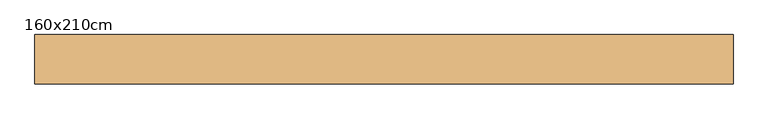
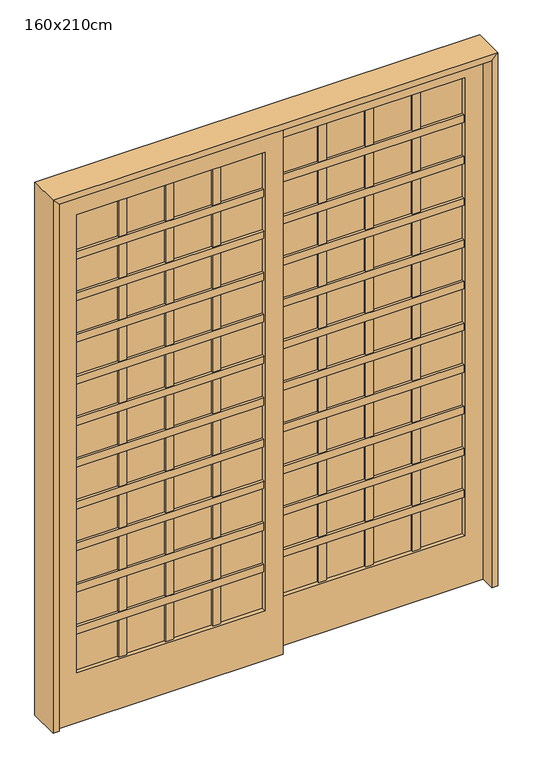
"""IFC4 building model written with IfcOpenShell, lengths in millimetres: door geometry, Porta de Correr Metálica Quadriculada : 160x210cm."""

from ifc_helpers import new_model, si_unit, frame, origin, place, context, project, spatial, polyline, outline, extrude, faceted_brep, source, transform, mapped, element, save


def door_160x210cm_3b8a9287(model_context):
    return source(origin(), model_context, "Body", "SolidModel", [
        extrude(outline(polyline([(-199.5, -52.1), (-199.5, -67.1101935), (-229.5, -67.1101935), (-229.5, -52.1), (-199.5, -52.1)])), frame((0.0, 0.0, 253.0), z_axis=(0.0, 0.0, 1.0), x_axis=(1.0, 0.0, 0.0)), (0.0, 0.0, 1.0), 1850.0),
        extrude(outline(polyline([(-379.0, -52.1), (-379.0, -67.1101935), (-409.0, -67.1101935), (-409.0, -52.1), (-379.0, -52.1)])), frame((0.0, 0.0, 253.0), z_axis=(0.0, 0.0, 1.0), x_axis=(1.0, 0.0, 0.0)), (0.0, 0.0, 1.0), 1850.0),
        extrude(outline(polyline([(-558.5, -52.1), (-558.5, -67.1101935), (-588.5, -67.1101935), (-588.5, -52.1), (-558.5, -52.1)])), frame((0.0, 0.0, 253.0), z_axis=(0.0, 0.0, 1.0), x_axis=(1.0, 0.0, 0.0)), (0.0, 0.0, 1.0), 1850.0),
        extrude(outline(polyline([(-35.0, -49.1), (-35.0, -70.1), (-753.0, -70.1), (-753.0, -49.1), (-35.0, -49.1)])), frame((0.0, 0.0, 1415.2727273), z_axis=(0.0, 0.0, 1.0), x_axis=(1.0, 0.0, 0.0)), (0.0, 0.0, 1.0), 30.0),
        extrude(outline(polyline([(-35.0, -49.1), (-35.0, -70.1), (-753.0, -70.1), (-753.0, -49.1), (-35.0, -49.1)])), frame((0.0, 0.0, 1247.0909091), z_axis=(0.0, 0.0, 1.0), x_axis=(1.0, 0.0, 0.0)), (0.0, 0.0, 1.0), 30.0),
        extrude(outline(polyline([(-35.0, -49.1), (-35.0, -70.1), (-753.0, -70.1), (-753.0, -49.1), (-35.0, -49.1)])), frame((0.0, 0.0, 1078.9090909), z_axis=(0.0, 0.0, 1.0), x_axis=(1.0, 0.0, 0.0)), (0.0, 0.0, 1.0), 30.0),
        extrude(outline(polyline([(-35.0, -49.1), (-35.0, -70.1), (-753.0, -70.1), (-753.0, -49.1), (-35.0, -49.1)])), frame((0.0, 0.0, 910.7272727), z_axis=(0.0, 0.0, 1.0), x_axis=(1.0, 0.0, 0.0)), (0.0, 0.0, 1.0), 30.0),
        extrude(outline(polyline([(-35.0, -49.1), (-35.0, -70.1), (-753.0, -70.1), (-753.0, -49.1), (-35.0, -49.1)])), frame((0.0, 0.0, 742.5454545), z_axis=(0.0, 0.0, 1.0), x_axis=(1.0, 0.0, 0.0)), (0.0, 0.0, 1.0), 30.0),
        extrude(outline(polyline([(-35.0, -49.1), (-35.0, -70.1), (-753.0, -70.1), (-753.0, -49.1), (-35.0, -49.1)])), frame((0.0, 0.0, 574.3636364), z_axis=(0.0, 0.0, 1.0), x_axis=(1.0, 0.0, 0.0)), (0.0, 0.0, 1.0), 30.0),
        extrude(outline(polyline([(-35.0, -49.1), (-35.0, -70.1), (-753.0, -70.1), (-753.0, -49.1), (-35.0, -49.1)])), frame((0.0, 0.0, 406.1818182), z_axis=(0.0, 0.0, 1.0), x_axis=(1.0, 0.0, 0.0)), (0.0, 0.0, 1.0), 30.0),
        extrude(outline(polyline([(-35.0, -49.1), (-35.0, -70.1), (-753.0, -70.1), (-753.0, -49.1), (-35.0, -49.1)])), frame((0.0, 0.0, 1919.8181818), z_axis=(0.0, 0.0, 1.0), x_axis=(1.0, 0.0, 0.0)), (0.0, 0.0, 1.0), 30.0),
        extrude(outline(polyline([(-35.0, -49.1), (-35.0, -70.1), (-753.0, -70.1), (-753.0, -49.1), (-35.0, -49.1)])), frame((0.0, 0.0, 1751.6363636), z_axis=(0.0, 0.0, 1.0), x_axis=(1.0, 0.0, 0.0)), (0.0, 0.0, 1.0), 30.0),
        extrude(outline(polyline([(-35.0, -49.1), (-35.0, -70.1), (-753.0, -70.1), (-753.0, -49.1), (-35.0, -49.1)])), frame((0.0, 0.0, 1583.4545455), z_axis=(0.0, 0.0, 1.0), x_axis=(1.0, 0.0, 0.0)), (0.0, 0.0, 1.0), 30.0),
        extrude(outline(polyline([(588.5, -10.1), (588.5, -25.1), (558.5, -25.1), (558.5, -10.1), (588.5, -10.1)])), frame((0.0, 0.0, 253.0), z_axis=(0.0, 0.0, 1.0), x_axis=(1.0, 0.0, 0.0)), (0.0, 0.0, 1.0), 1850.0),
        extrude(outline(polyline([(409.0, -10.1), (409.0, -25.1), (379.0, -25.1), (379.0, -10.1), (409.0, -10.1)])), frame((0.0, 0.0, 253.0), z_axis=(0.0, 0.0, 1.0), x_axis=(1.0, 0.0, 0.0)), (0.0, 0.0, 1.0), 1850.0),
        extrude(outline(polyline([(229.5, -10.1), (229.5, -25.1), (199.5, -25.1), (199.5, -10.1), (229.5, -10.1)])), frame((0.0, 0.0, 253.0), z_axis=(0.0, 0.0, 1.0), x_axis=(1.0, 0.0, 0.0)), (0.0, 0.0, 1.0), 1850.0),
        extrude(outline(polyline([(753.0, -7.1), (753.0, -28.1), (35.0, -28.1), (35.0, -7.1), (753.0, -7.1)])), frame((0.0, 0.0, 1415.2727273), z_axis=(0.0, 0.0, 1.0), x_axis=(1.0, 0.0, 0.0)), (0.0, 0.0, 1.0), 30.0),
        extrude(outline(polyline([(753.0, -7.1), (753.0, -28.1), (35.0, -28.1), (35.0, -7.1), (753.0, -7.1)])), frame((0.0, 0.0, 1247.0909091), z_axis=(0.0, 0.0, 1.0), x_axis=(1.0, 0.0, 0.0)), (0.0, 0.0, 1.0), 30.0),
        extrude(outline(polyline([(753.0, -7.1), (753.0, -28.1), (35.0, -28.1), (35.0, -7.1), (753.0, -7.1)])), frame((0.0, 0.0, 1078.9090909), z_axis=(0.0, 0.0, 1.0), x_axis=(1.0, 0.0, 0.0)), (0.0, 0.0, 1.0), 30.0),
        extrude(outline(polyline([(753.0, -7.1), (753.0, -28.1), (35.0, -28.1), (35.0, -7.1), (753.0, -7.1)])), frame((0.0, 0.0, 910.7272727), z_axis=(0.0, 0.0, 1.0), x_axis=(1.0, 0.0, 0.0)), (0.0, 0.0, 1.0), 30.0),
        extrude(outline(polyline([(753.0, -7.1), (753.0, -28.1), (35.0, -28.1), (35.0, -7.1), (753.0, -7.1)])), frame((0.0, 0.0, 742.5454545), z_axis=(0.0, 0.0, 1.0), x_axis=(1.0, 0.0, 0.0)), (0.0, 0.0, 1.0), 30.0),
        extrude(outline(polyline([(753.0, -7.1), (753.0, -28.1), (35.0, -28.1), (35.0, -7.1), (753.0, -7.1)])), frame((0.0, 0.0, 574.3636364), z_axis=(0.0, 0.0, 1.0), x_axis=(1.0, 0.0, 0.0)), (0.0, 0.0, 1.0), 30.0),
        extrude(outline(polyline([(753.0, -7.1), (753.0, -28.1), (35.0, -28.1), (35.0, -7.1), (753.0, -7.1)])), frame((0.0, 0.0, 406.1818182), z_axis=(0.0, 0.0, 1.0), x_axis=(1.0, 0.0, 0.0)), (0.0, 0.0, 1.0), 30.0),
        extrude(outline(polyline([(753.0, -7.1), (753.0, -28.1), (35.0, -28.1), (35.0, -7.1), (753.0, -7.1)])), frame((0.0, 0.0, 1919.8181818), z_axis=(0.0, 0.0, 1.0), x_axis=(1.0, 0.0, 0.0)), (0.0, 0.0, 1.0), 30.0),
        extrude(outline(polyline([(753.0, -7.1), (753.0, -28.1), (35.0, -28.1), (35.0, -7.1), (753.0, -7.1)])), frame((0.0, 0.0, 1751.6363636), z_axis=(0.0, 0.0, 1.0), x_axis=(1.0, 0.0, 0.0)), (0.0, 0.0, 1.0), 30.0),
        extrude(outline(polyline([(753.0, -7.1), (753.0, -28.1), (35.0, -28.1), (35.0, -7.1), (753.0, -7.1)])), frame((0.0, 0.0, 1583.4545455), z_axis=(0.0, 0.0, 1.0), x_axis=(1.0, 0.0, 0.0)), (0.0, 0.0, 1.0), 30.0),
        extrude(outline(polyline([(2173.0, -35.0), (53.0, -35.0), (53.0, 823.0), (2173.0, 823.0), (2173.0, -35.0)]), holes=[polyline([(2103.0, 35.0), (2103.0, 753.0), (253.0, 753.0), (253.0, 35.0), (2103.0, 35.0)])]), frame((0.0, -33.6, 0.0), z_axis=(0.0, 1.0, 0.0), x_axis=(0.0, 0.0, 1.0)), (0.0, 0.0, 1.0), 32.0),
        faceted_brep([(-826.0, -85.6, 50.0), (-850.0, -85.6, 50.0), (-850.0, 34.4, 50.0), (-826.0, 34.4, 50.0), (-826.0, 34.4, 2176.0), (-826.0, -85.6, 2176.0), (-850.0, 34.4, 2200.0), (-850.0, -85.6, 2200.0), (826.0, -85.6, 50.0), (826.0, 34.4, 50.0), (850.0, 34.4, 50.0), (850.0, -85.6, 50.0), (826.0, -85.6, 2176.0), (850.0, -85.6, 2200.0), (850.0, 34.4, 2200.0), (826.0, 34.4, 2176.0)], [[[0, 1, 2, 3]], [[3, 4, 5, 0]], [[2, 6, 4, 3]], [[1, 7, 6, 2]], [[0, 5, 7, 1]], [[8, 9, 10, 11]], [[12, 8, 11, 13]], [[13, 11, 10, 14]], [[14, 10, 9, 15]], [[15, 9, 8, 12]], [[4, 15, 12, 5]], [[6, 14, 15, 4]], [[7, 13, 14, 6]], [[5, 12, 13, 7]]]),
        extrude(outline(polyline([(2173.0, -823.0), (53.0, -823.0), (53.0, 35.0), (2173.0, 35.0), (2173.0, -823.0)]), holes=[polyline([(2103.0, -753.0), (2103.0, -35.0), (253.0, -35.0), (253.0, -753.0), (2103.0, -753.0)])]), frame((0.0, -75.6, 0.0), z_axis=(0.0, 1.0, 0.0), x_axis=(0.0, 0.0, 1.0)), (0.0, 0.0, 1.0), 32.0),
        extrude(outline(polyline([(-35.0, -54.1), (-35.0, -60.1), (-753.0, -60.1), (-753.0, -54.1), (-35.0, -54.1)])), frame((0.0, 0.0, 253.0), z_axis=(0.0, 0.0, 1.0), x_axis=(1.0, 0.0, 0.0)), (0.0, 0.0, 1.0), 1850.0),
        extrude(outline(polyline([(753.0, -12.1), (753.0, -18.1), (35.0, -18.1), (35.0, -12.1), (753.0, -12.1)])), frame((0.0, 0.0, 253.0), z_axis=(0.0, 0.0, 1.0), x_axis=(1.0, 0.0, 0.0)), (0.0, 0.0, 1.0), 1850.0),
    ])


if __name__ == "__main__":
    model = new_model("IFC4")
    model_context = context("Model", 3, world=origin())
    ifc_project = project(units=[si_unit("LENGTHUNIT", "METRE", prefix="MILLI")], contexts=[model_context])
    site = spatial("IfcSite", under=ifc_project)
    building = spatial("IfcBuilding", under=site)
    placement = place(None, origin())
    door_160x210cm_shape = door_160x210cm_3b8a9287(model_context)
    element("IfcDoor", 1, ObjectType="Porta de Correr Metálica Quadriculada : 160x210cm", at=placement, inside=building, context=model_context, shape_type="MappedRepresentation", body=[
        mapped(door_160x210cm_shape, transform((0.0, 0.0, 0.0), x_axis=(1.0, 0.0, 0.0), y_axis=(0.0, 1.0, 0.0), z_axis=(0.0, 0.0, 1.0))),
    ])
    save(model, "model.ifc")

# Revit data of these elements
# Type "Porta de Correr Metálica Quadriculada : 160x210cm"
#   Type Mark = ""
#   SINAPI = ""
#   Construction Type = "300"
#   Maçaneta [instance default] = ""
#   Fechadura [instance default] = ""
#   Vão Luz (somente para informação) = 163.20 cm
#   Tolerância Folha Vertical = 0.30 cm
#   Módulo Básico M = 10.00 cm
#   Largura de Coordenação Modular Largura CM = 170.00 cm
#   Rough Width = 170.00 cm
#   Largura Vidro = 71.80 cm
#   Altura de Coordenação Modular Largura CM = 220.00 cm
#   Rough Height = 220.00 cm
#   Altura Nominal = 211.60 cm
#   Ajuste de Coordenação Topo AC Topo = 0.00 cm
#   Ajuste de Coordenação Base AC Base = 5.00 cm
#   Ajuste de Coordenação AC = 0.00 cm
#   Tolerância Folha Horizontal = 0.30 cm
#   Largura Folha somente para informação = 85.80 cm
#   Espessura Folha = 3.20 cm
#   Maçaneta - Distância da Folha = 3.40 cm
#   Maçaneta - Altura = 100.00 cm
#   Largura Nominal (Largura Mn) = 165.20 cm
#   Distância do Nível = 0.30 cm
#   Aduela Interna Espessura = 2.40 cm
#   Aduela Externa Espessura = 3.40 cm
#   Altura Folha somente para informação = 212.00 cm
#   Height = 215.00 cm
#   Width = 170.00 cm
#   Número de Módulos Básicos nM Largura = 17
#   Número de Módulos Básicos nM Altura = 22
#   Aduela Metálica de Canto = no
#   Vidro - Material = Vidro
#   Batente - Material [instance default] = none
#   Painel - Material [instance default] = none
#   Model = ""
#   Function = (empty or 0)
#   Description = (empty or 0)
#   Wall Closure = (empty or 0)
#   Assembly Code = ""
# Element 1 (IfcDoor, "Porta de Correr Metálica Quadriculada : 160x210cm")
#   Materials on its faces: "Vidro"
# Materials
#   "Vidro": class "Vidro", colour RGB 230 230 230, transparency 0.75, Cost = 0
